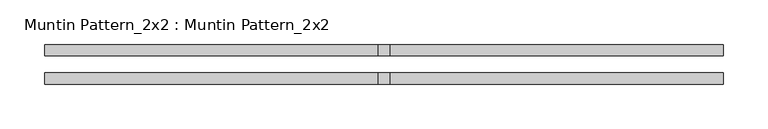
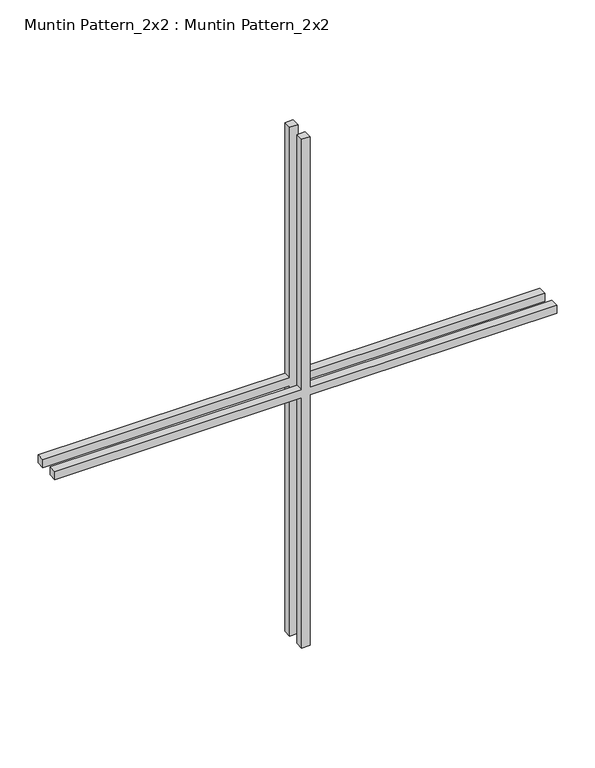
"""IFC4 building model written with IfcOpenShell, lengths in millimetres: proxy geometry, Muntin Pattern_2x2 : Muntin Pattern_2x2."""

import ifcopenshell
import ifcopenshell.guid

model = None  # the IFC model being written
_history = None  # IfcOwnerHistory: only IFC2X3 demands one
_inside = {}  # id of a spatial element -> (the spatial element, [elements in it])
_under = {}  # id of a project, library or spatial element -> (it, [spatial elements below it])
_declared = {}  # id of a project -> (the project, [libraries it declares])
_typed = {}  # id of a type object -> (the type object, [elements of that type])
_made_of = {}  # id of a material, layer set ... -> (it, [elements and type objects made of it])


def new_model(schema):
    """Start an empty IFC model of exactly this schema.

    Asked for "IFC4X3", IfcOpenShell would pick the latest addendum, in which some entities
    have other attributes; the version numbers below select the first issue.
    IFC2X3 requires an IfcOwnerHistory on every rooted entity: one is made here for all.
    """
    global model, _history
    if schema == "IFC4X3":
        model = ifcopenshell.file(schema_version=(4, 3, 0, 0))
    else:
        model = ifcopenshell.file(schema=schema)
    _inside.clear()
    _under.clear()
    _declared.clear()
    _typed.clear()
    _made_of.clear()
    _history = None
    if model.schema == "IFC2X3":
        org = make("IfcOrganization", Name="unknown")
        user = make(
            "IfcPersonAndOrganization",
            ThePerson=make("IfcPerson", FamilyName="unknown"),
            TheOrganization=org,
        )
        app = make(
            "IfcApplication",
            ApplicationDeveloper=org,
            Version="unknown",
            ApplicationFullName="unknown",
            ApplicationIdentifier="unknown",
        )
        _history = make(
            "IfcOwnerHistory",
            OwningUser=user,
            OwningApplication=app,
            ChangeAction="ADDED",
            CreationDate=0,
        )
    return model


def make(cls, **values):
    """One entity of the class cls with the attributes given. An attribute that is None is left unset."""
    return model.create_entity(
        cls, **{name: value for name, value in values.items() if value is not None}
    )


def rooted(cls, **values):
    """An entity with a GlobalId (a new one), such as an element, a storey or a relation."""
    return make(cls, GlobalId=ifcopenshell.guid.new(), OwnerHistory=_history, **values)


def si_unit(unit_type, name, prefix=None):
    """IfcSIUnit, for example si_unit("LENGTHUNIT", "METRE", prefix="MILLI")."""
    return make("IfcSIUnit", UnitType=unit_type, Prefix=prefix, Name=name)


def assignment(units):
    """IfcUnitAssignment: the units of a project."""
    return None if units is None else make("IfcUnitAssignment", Units=units)


def point(xyz):
    """IfcCartesianPoint."""
    return None if xyz is None else make("IfcCartesianPoint", Coordinates=xyz)


def direction(xyz):
    """IfcDirection."""
    return None if xyz is None else make("IfcDirection", DirectionRatios=xyz)


def frame(location, z_axis=None, x_axis=None):
    """IfcAxis2Placement3D, a coordinate frame: its origin and axes. An axis left out is left unset."""
    return make(
        "IfcAxis2Placement3D",
        Location=point(location),
        Axis=direction(z_axis),
        RefDirection=direction(x_axis),
    )


def origin():
    """The frame at (0, 0, 0) with its axes left unset."""
    return frame((0.0, 0.0, 0.0))


def place(relative_to, where):
    """IfcLocalPlacement: puts the frame where relative to a parent placement (None: the world)."""
    return make(
        "IfcLocalPlacement", PlacementRelTo=relative_to, RelativePlacement=where
    )


def context(
    kind, dimensions, precision=None, world=None, true_north=None, identifier=None
):
    """IfcGeometricRepresentationContext, for example the 3D "Model" context."""
    return make(
        "IfcGeometricRepresentationContext",
        ContextIdentifier=identifier,
        ContextType=kind,
        CoordinateSpaceDimension=dimensions,
        Precision=precision,
        WorldCoordinateSystem=world,
        TrueNorth=true_north,
    )


def project(units=None, contexts=None):
    """IfcProject with its units and contexts."""
    return rooted(
        "IfcProject",
        Name="project",
        RepresentationContexts=contexts,
        UnitsInContext=assignment(units),
    )


def spatial(cls, under=None, at=None, **own):
    """A site, building, storey or space (cls), placed at a placement, below another one or the project."""
    s = rooted(cls, ObjectPlacement=at, **own)
    if under is not None:
        _under.setdefault(under.id(), (under, []))[1].append(s)
    return s


def polyline(points):
    """IfcPolyline through the points."""
    return make("IfcPolyline", Points=[point(p) for p in points])


def outline(outer, holes=None, kind="AREA"):
    """IfcArbitraryClosedProfileDef: a profile drawn as a closed curve; with holes, ...WithVoids."""
    if holes is None:
        return make("IfcArbitraryClosedProfileDef", ProfileType=kind, OuterCurve=outer)
    return make(
        "IfcArbitraryProfileDefWithVoids",
        ProfileType=kind,
        OuterCurve=outer,
        InnerCurves=holes,
    )


def extrude(swept, where, along, depth):
    """IfcExtrudedAreaSolid: the profile swept, set in the frame where, extruded along a direction by depth."""
    return make(
        "IfcExtrudedAreaSolid",
        SweptArea=swept,
        Position=where,
        ExtrudedDirection=direction(along),
        Depth=depth,
    )


def shape(context_of_items, identifier, shape_type, items):
    """IfcShapeRepresentation: the items that make up one representation, for example the "Body"."""
    return make(
        "IfcShapeRepresentation",
        ContextOfItems=context_of_items,
        RepresentationIdentifier=identifier,
        RepresentationType=shape_type,
        Items=items,
    )


def source(mapping_origin, context_of_items, identifier, shape_type, items):
    """IfcRepresentationMap: a shape defined once, which mapped items show again and again."""
    return make(
        "IfcRepresentationMap",
        MappingOrigin=mapping_origin,
        MappedRepresentation=shape(context_of_items, identifier, shape_type, items),
    )


def transform(
    local_origin,
    x_axis=None,
    y_axis=None,
    z_axis=None,
    scale=None,
    scale2=None,
    scale3=None,
    uniform=True,
):
    """IfcCartesianTransformationOperator3D, or its non-uniform kind. x_axis, y_axis, z_axis: its Axis1, 2, 3."""
    if uniform:
        return make(
            "IfcCartesianTransformationOperator3D",
            Axis1=direction(x_axis),
            Axis2=direction(y_axis),
            LocalOrigin=point(local_origin),
            Scale=scale,
            Axis3=direction(z_axis),
        )
    return make(
        "IfcCartesianTransformationOperator3DnonUniform",
        Axis1=direction(x_axis),
        Axis2=direction(y_axis),
        LocalOrigin=point(local_origin),
        Scale=scale,
        Axis3=direction(z_axis),
        Scale2=scale2,
        Scale3=scale3,
    )


def mapped(mapping_source, mapping_target):
    """IfcMappedItem: shows the shape of a source again, moved by a transform."""
    return make(
        "IfcMappedItem", MappingSource=mapping_source, MappingTarget=mapping_target
    )


def made_of(thing, what):
    """Note that an element or type object is made of a material, layer set ...; save() writes the relation."""
    if what is not None:
        _made_of.setdefault(what.id(), (what, []))[1].append(thing)
    return thing


def element(
    cls,
    number,
    at=None,
    inside=None,
    cuts=None,
    type_object=None,
    material=None,
    context=None,
    identifier="Body",
    shape_type=None,
    held_by="IfcProductDefinitionShape",
    body=None,
    shapes=None,
    **own,
):
    """One element of the class cls, such as IfcWall. Its Tag is "e" and its number.

    at: its placement. inside: the storey or other place that contains it. cuts: it is an
    opening in that element (IfcRelVoidsElement). A single representation is given by context,
    identifier, shape_type and body (its items); several are given by shapes. held_by: the class
    of the entity that holds the representations. save() writes the other relations.
    """
    e = rooted(cls, Tag="e%d" % number, ObjectPlacement=at, **own)
    if body is not None:
        shapes = [shape(context, identifier, shape_type, body)]
    if shapes is not None:
        e.Representation = make(held_by, Representations=shapes)
    if inside is not None:
        _inside.setdefault(inside.id(), (inside, []))[1].append(e)
    if cuts is not None:
        rooted(
            "IfcRelVoidsElement", RelatingBuildingElement=cuts, RelatedOpeningElement=e
        )
    if type_object is not None:
        _typed.setdefault(type_object.id(), (type_object, []))[1].append(e)
    return made_of(e, material)


def aggregate(whole, parts):
    """IfcRelAggregates: a whole, such as a stair, and the parts it consists of."""
    return rooted("IfcRelAggregates", RelatingObject=whole, RelatedObjects=parts)


def save(model, path):
    """Write the relations noted so far, then the file.

    IfcRelAggregates (storeys below a building ...), IfcRelContainedInSpatialStructure (elements
    in a storey), IfcRelDefinesByType, IfcRelAssociatesMaterial and IfcRelDeclares: one each for
    every whole, place, type object, material and project.
    """
    for whole, parts in _under.values():
        aggregate(whole, parts)
    for where, things in _inside.values():
        rooted(
            "IfcRelContainedInSpatialStructure",
            RelatedElements=things,
            RelatingStructure=where,
        )
    for kind, things in _typed.values():
        rooted("IfcRelDefinesByType", RelatedObjects=things, RelatingType=kind)
    for what, things in _made_of.values():
        rooted("IfcRelAssociatesMaterial", RelatedObjects=things, RelatingMaterial=what)
    for by, libraries in _declared.values():
        rooted("IfcRelDeclares", RelatingContext=by, RelatedDefinitions=libraries)
    model.write(path)


def muntin_pattern_2x2_muntin_pattern_2x2_74d79337(model_context):
    return source(origin(), model_context, "Body", "SweptSolid", [
        extrude(outline(polyline([(414.3375, -6.35), (414.3375, -381.0), (401.6375, -381.0), (401.6375, -6.35), (0.0, -6.35), (0.0, 6.35), (401.6375, 6.35), (401.6375, 381.0), (414.3375, 381.0), (414.3375, 6.35), (815.975, 6.35), (815.975, -6.35), (414.3375, -6.35)])), frame((0.0, -22.225, 0.0), z_axis=(0.0, 1.0, 0.0), x_axis=(0.0, 0.0, 1.0)), (0.0, 0.0, 1.0), 12.7),
        extrude(outline(polyline([(414.3375, -6.35), (414.3375, -381.0), (401.6375, -381.0), (401.6375, -6.35), (0.0, -6.35), (0.0, 6.35), (401.6375, 6.35), (401.6375, 381.0), (414.3375, 381.0), (414.3375, 6.35), (815.975, 6.35), (815.975, -6.35), (414.3375, -6.35)])), frame((0.0, 9.525, 0.0), z_axis=(0.0, 1.0, 0.0), x_axis=(0.0, 0.0, 1.0)), (0.0, 0.0, 1.0), 12.7),
    ])


if __name__ == "__main__":
    model = new_model("IFC4")
    model_context = context("Model", 3, world=origin())
    ifc_project = project(units=[si_unit("LENGTHUNIT", "METRE", prefix="MILLI")], contexts=[model_context])
    site = spatial("IfcSite", under=ifc_project)
    building = spatial("IfcBuilding", under=site)
    placement = place(None, origin())
    muntin_pattern_2x2_muntin_pattern_2x2_shape = muntin_pattern_2x2_muntin_pattern_2x2_74d79337(model_context)
    element("IfcBuildingElementProxy", 1, Name="Muntin Pattern_2x2 : Muntin Pattern_2x2", ObjectType="Muntin Pattern_2x2 : Muntin Pattern_2x2", at=placement, inside=building, context=model_context, shape_type="MappedRepresentation", body=[
        mapped(muntin_pattern_2x2_muntin_pattern_2x2_shape, transform((0.0, 0.0, 0.0), x_axis=(1.0, 0.0, 0.0), y_axis=(0.0, 1.0, 0.0), z_axis=(0.0, 0.0, 1.0))),
    ])
    save(model, "model.ifc")

# Revit data of these elements
# Type "Muntin Pattern_2x2 : Muntin Pattern_2x2"
#   Width [instance default] = 4' - 0"
#   Thickness = 0' - 0 1/2"
#   Height [instance default] = 4' - 0"
#   Distance = 0' - 0 3/4"
#   Interior Material [instance default] = none
#   Exterior Material [instance default] = none
#   Default Elevation = 0
# Element 1 (IfcBuildingElementProxy, "Muntin Pattern_2x2 : Muntin Pattern_2x2")
#   Width = 2' - 6"
#   Height = 2' - 8 1/8"
#   Interior Material = Wood - Stained
#   Exterior Material = Clad - White
#   Materials on its faces: "Clad - White", "Wood - Stained"
# Materials
#   "Clad - White": class "Wood", colour RGB 242 242 238, transparency 0, Cost = 0
#   "Wood - Stained": class "Wood", colour RGB 224 178 126, transparency 0, Cost = 0
